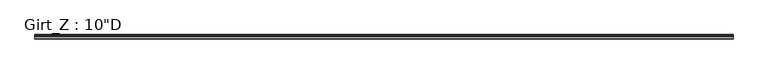
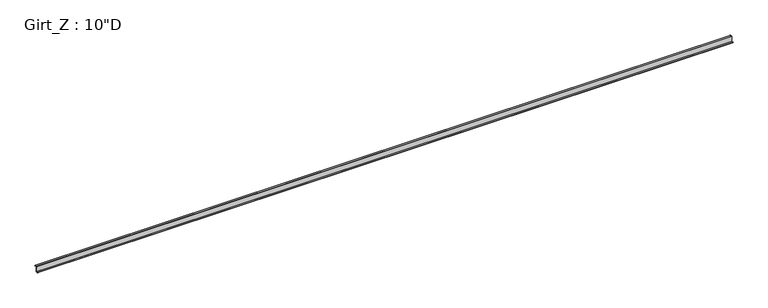
"""IFC4 building model written with IfcOpenShell, lengths in millimetres: beam geometry."""

from ifc_helpers import new_model, si_unit, point, frame, frame_2d, origin, place, context, project, spatial, polyline, circle_curve, trimmed, segment, composite_curve, outline, extrude, source, transform, mapped, element, save


def beam_ace1880b(model_context):
    return source(origin(), model_context, "Body", "SweptSolid", [
        extrude(outline(composite_curve([segment(polyline([(77.9859375, 127.0), (90.2310415, 112.4068534), (88.1028742, 110.621109), (76.6904765, 124.221875), (3.3005807, 124.221875)]), True, "CONTINUOUS"), segment(trimmed(circle_curve(frame_2d((3.3741066, 122.2381931)), 1.9850441), [point((3.3005807, 124.221875))], [point((1.3890625, 122.2381931))], True, "CARTESIAN"), True, "CONTINUOUS"), segment(polyline([(1.3890625, 122.2381931), (1.3890625, -127.0), (-84.3359375, -127.0), (-96.5810415, -112.4068534), (-94.4528742, -110.621109), (-83.0404765, -124.221875), (-3.2694106, -124.221875)]), True, "CONTINUOUS"), segment(trimmed(circle_curve(frame_2d((-3.3748024, -122.2389339)), 1.9857399), [point((-3.2694106, -124.221875))], [point((-1.3890625, -122.2389339))], True, "CARTESIAN"), True, "CONTINUOUS"), segment(polyline([(-1.3890625, -122.2389339), (-1.3890625, 122.2375)]), True, "CONTINUOUS"), segment(trimmed(circle_curve(frame_2d((3.3734375, 122.2375)), 4.7625), [point((-1.3890625, 122.2375))], [point((3.3734375, 127.0))], False, "CARTESIAN"), True, "CONTINUOUS"), segment(polyline([(3.3734375, 127.0), (77.9859375, 127.0)]), True, "CONTINUOUS")], self_intersect=False)), frame((-15560.675, 0.0, 0.0), z_axis=(1.0, 0.0, 0.0), x_axis=(0.0, 1.0, 0.0)), (0.0, 0.0, 1.0), 31121.35),
    ])


if __name__ == "__main__":
    model = new_model("IFC4")
    model_context = context("Model", 3, world=origin())
    ifc_project = project(units=[si_unit("LENGTHUNIT", "METRE", prefix="MILLI")], contexts=[model_context])
    site = spatial("IfcSite", under=ifc_project)
    building = spatial("IfcBuilding", under=site)
    placement = place(None, origin())
    beam_shape = beam_ace1880b(model_context)
    element("IfcBeam", 1, ObjectType="Girt_Z : 10\"D", at=placement, inside=building, context=model_context, shape_type="MappedRepresentation", body=[
        mapped(beam_shape, transform((0.0, 0.0, 0.0), x_axis=(1.0, 0.0, 0.0), y_axis=(0.0, 1.0, 0.0), z_axis=(0.0, 0.0, 1.0))),
    ])
    save(model, "model.ifc")

# Revit data of these elements
# Type "Girt_Z : 10\"D"
#   half leg = 0' - 1 11/16"
#   Web_Thickness = 0' - 0 7/64"
#   Length [instance default] = 10' - 0"
#   Leg_2 = 0' - 3 3/8"
#   Leg_1 = 0' - 3 1/8"
#   Height = 0' - 10"
#   Structural Material [instance default] = none
# Element 1 (IfcBeam, "Girt_Z : 10\"D")
#   Structural Material = STRUCTURAL STEEL - SEE STRUCT. DWGS
#   Materials on its faces: "STRUCTURAL STEEL - SEE STRUCT. DWGS"
# Materials
#   "STRUCTURAL STEEL - SEE STRUCT. DWGS": class "Metal", colour RGB 137 146 153, transparency 0, Description = "Steel, mill finish", Cost = 0
